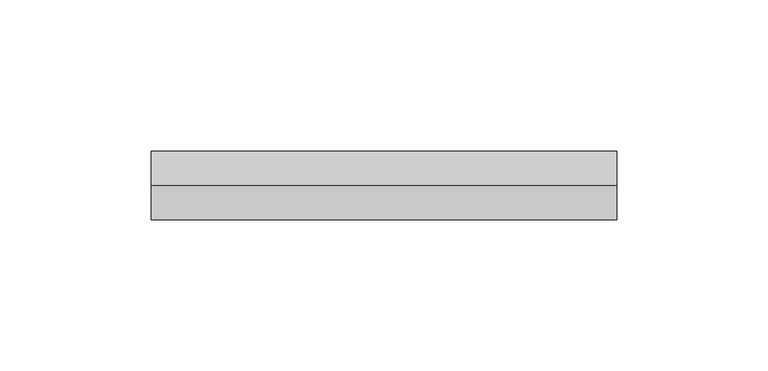
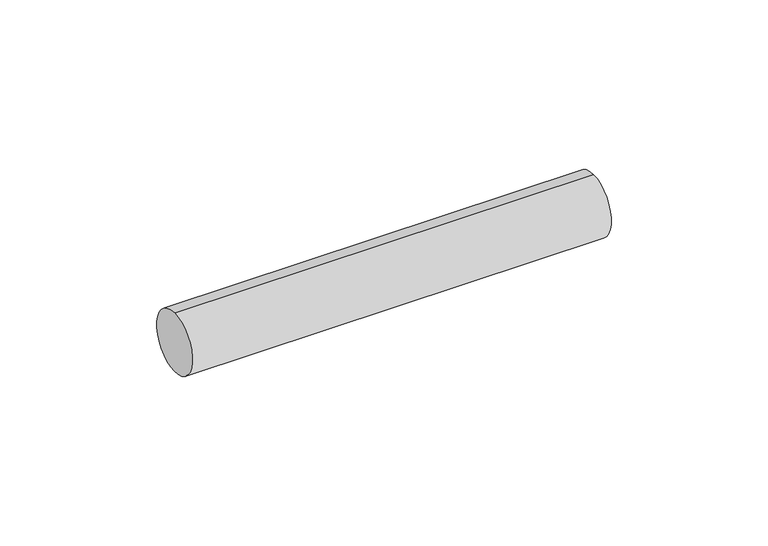
"""IFC4 building model written with IfcOpenShell, lengths in millimetres: proxy geometry, Bolt20:Bolt003:304690 : Bolt20:Bolt003:304690."""

from ifc_helpers import new_model, si_unit, point, frame, frame_2d, origin, place, context, project, spatial, circle_curve, trimmed, segment, composite_curve, outline, extrude, source, transform, mapped, element, save


def generic_models_9930d7c8(model_context):
    return source(origin(), model_context, "Body", "SweptSolid", [
        extrude(outline(composite_curve([segment(trimmed(circle_curve(frame_2d((2174.9207483, 40070.0545241)), 11.4045168), [point((2174.9207483, 40058.6500073))], [point((2174.9207483, 40081.4590409))], False, "CARTESIAN"), True, "CONTINUOUS"), segment(trimmed(circle_curve(frame_2d((2174.9207483, 40070.0545241)), 11.4045168), [point((2174.9207483, 40081.4590409))], [point((2174.9207483, 40058.6500073))], False, "CARTESIAN"), True, "CONTINUOUS")], self_intersect=False)), frame((15064.3231907, 0.0, 0.0), z_axis=(1.0, 0.0, 0.0), x_axis=(0.0, 1.0, 0.0)), (0.0, 0.0, 1.0), 154.0602393),
    ])


if __name__ == "__main__":
    model = new_model("IFC4")
    model_context = context("Model", 3, world=origin())
    ifc_project = project(units=[si_unit("LENGTHUNIT", "METRE", prefix="MILLI")], contexts=[model_context])
    site = spatial("IfcSite", under=ifc_project)
    building = spatial("IfcBuilding", under=site)
    placement = place(None, origin())
    generic_models_shape = generic_models_9930d7c8(model_context)
    element("IfcBuildingElementProxy", 1, Name="Bolt20:Bolt003:304690 : Bolt20:Bolt003:304690", ObjectType="Bolt20:Bolt003:304690 : Bolt20:Bolt003:304690", at=placement, inside=building, context=model_context, shape_type="MappedRepresentation", body=[
        mapped(generic_models_shape, transform((0.0, 0.0, 0.0), x_axis=(1.0, 0.0, 0.0), y_axis=(0.0, 1.0, 0.0), z_axis=(0.0, 0.0, 1.0))),
    ])
    save(model, "model.ifc")

# Revit data of these elements
# Type "Bolt20:Bolt003:304690 : Bolt20:Bolt003:304690"
#   NameOverride = "Bolt20:Bolt003:304690"
#   ObjectTypeOverride = "Bolt20:Bolt003"
#   Reference = "Bolt003"
#   Category = "Generic Models"
#   Tag = "304690"
# Element 1 (IfcBuildingElementProxy, "Bolt20:Bolt003:304690 : Bolt20:Bolt003:304690")
#   Materials on its faces: "TUBE STEEL STRINGER WELDED TO ANCHORED STEEL PLATE - SEE STRUCT DWGS"
# Materials
#   "TUBE STEEL STRINGER WELDED TO ANCHORED STEEL PLATE - SEE STRUCT DWGS": class "Unassigned", colour RGB 128 128 128, transparency 0, Cost = 0
